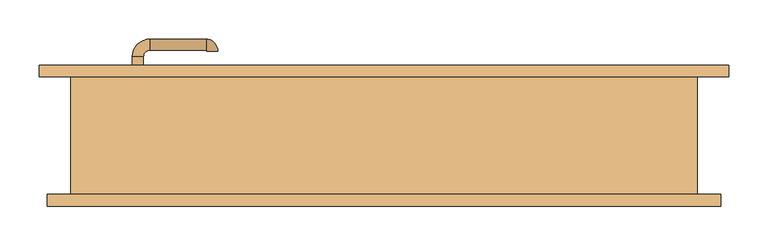
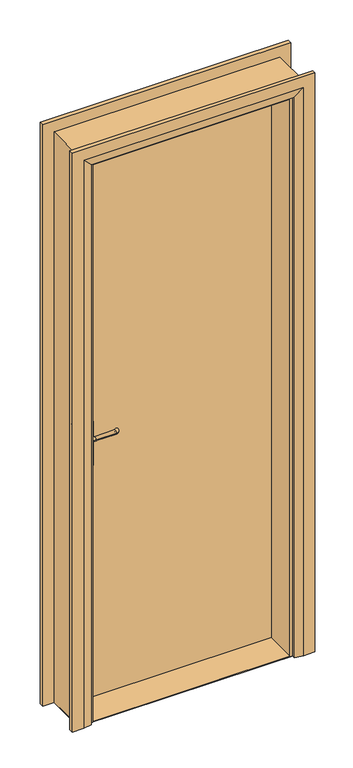
"""IFC4 building model written with IfcOpenShell, lengths in millimetres: door geometry, Porta Simples de Abrir : 70x210cm - Marco de Madeira."""

from ifc_helpers import new_model, si_unit, point, frame, frame_2d, origin, place, context, project, spatial, polyline, circle_curve, ellipse_curve, trimmed, segment, composite_curve, outline, extrude, faceted_brep, source, transform, mapped, element, save
from ifc_brep_helpers import plane_surface, cylinder_surface, revolved_surface, advanced_brep


def door_49983123(model_context):
    return source(origin(), model_context, "Body", "SolidModel", [
        extrude(outline(composite_curve([segment(trimmed(circle_curve(frame_2d((1050.0, -314.0)), 20.0), [point((1050.0, -334.0))], [point((1050.0, -294.0))], False, "CARTESIAN"), True, "CONTINUOUS"), segment(trimmed(circle_curve(frame_2d((1050.0, -314.0)), 20.0), [point((1050.0, -294.0))], [point((1050.0, -334.0))], False, "CARTESIAN"), True, "CONTINUOUS")], self_intersect=False)), frame((0.0, 29.4070105, 0.0), z_axis=(0.0, 1.0, 0.0), x_axis=(0.0, 0.0, 1.0)), (0.0, 0.0, 1.0), 4.5929895),
        advanced_brep(
        [(-307.0, 29.4070105, 1050.0), (-321.0, 29.4070105, 1050.0), (-321.0, 14.0, 1050.0), (-307.0, 14.0, 1050.0), (-299.0, -8.0, 1050.0), (-299.0, 6.0, 1050.0), (-227.0, -8.0, 1050.0), (-227.0, 6.0, 1050.0), (-226.0, 7.0, 1050.0), (-212.0, 7.0, 1050.0)],
        [
            (0, 1, circle_curve(frame((-314.0, 29.4070105, 1050.0), z_axis=(0.0, 1.0, 0.0), x_axis=(-1.0, 0.0, 0.0)), 7.0)),
            (1, 0, circle_curve(frame((-314.0, 29.4070105, 1050.0), z_axis=(0.0, 1.0, 0.0), x_axis=(-1.0, 0.0, 0.0)), 7.0)),
            (1, 2),
            (2, 3, circle_curve(frame((-314.0, 14.0, 1050.0), z_axis=(0.0, 1.0, 0.0), x_axis=(-1.0, 0.0, 0.0)), 7.0)),
            (3, 0),
            (3, 2, circle_curve(frame((-314.0, 14.0, 1050.0), z_axis=(0.0, 1.0, 0.0), x_axis=(-1.0, 0.0, 0.0)), 7.0)),
            (4, 5, circle_curve(frame((-299.0, -1.0, 1050.0), z_axis=(-1.0, 0.0, 0.0), x_axis=(0.0, -1.0, 0.0)), 7.0)),
            (5, 3, circle_curve(frame((-299.0, 14.0, 1050.0), z_axis=(0.0, 0.0, -1.0), x_axis=(-1.0, 0.0, 0.0)), 8.0)),
            (2, 4, circle_curve(frame((-299.0, 14.0, 1050.0), z_axis=(0.0, 0.0, 1.0), x_axis=(-1.0, 0.0, 0.0)), 22.0)),
            (5, 4, circle_curve(frame((-299.0, -1.0, 1050.0), z_axis=(-1.0, 0.0, 0.0), x_axis=(0.0, -1.0, 0.0)), 7.0)),
            (4, 6),
            (6, 7, circle_curve(frame((-227.0, -1.0, 1050.0), z_axis=(-1.0, 0.0, 0.0), x_axis=(0.0, -1.0, 0.0)), 7.0)),
            (7, 5),
            (7, 6, circle_curve(frame((-227.0, -1.0, 1050.0), z_axis=(-1.0, 0.0, 0.0), x_axis=(0.0, -1.0, 0.0)), 7.0)),
            (8, 9, circle_curve(frame((-219.0, 7.0, 1050.0), z_axis=(0.0, 1.0, 0.0), x_axis=(1.0, 0.0, 0.0)), 7.0)),
            (9, 8, circle_curve(frame((-219.0, 7.0, 1050.0), z_axis=(0.0, 1.0, 0.0), x_axis=(1.0, 0.0, 0.0)), 7.0)),
            (8, 7, circle_curve(frame((-227.0, 7.0, 1050.0), z_axis=(0.0, 0.0, -1.0), x_axis=(0.0, -1.0, 0.0)), 1.0)),
            (6, 9, circle_curve(frame((-227.0, 7.0, 1050.0), z_axis=(0.0, 0.0, 1.0), x_axis=(0.0, -1.0, 0.0)), 15.0)),
        ],
        [
            plane_surface(frame((-314.0, 29.4070105, 1050.0), z_axis=(0.0, 1.0, 0.0), x_axis=(0.0, 0.0, 1.0))),
            cylinder_surface(frame((-314.0, 29.4070105, 1050.0), z_axis=(0.0, 1.0, 0.0), x_axis=(-1.0, 0.0, 0.0)), 7.0),
            revolved_surface(trimmed(ellipse_curve(frame((-314.0, 14.0, 1050.0), z_axis=(0.0, -1.0, 0.0), x_axis=(-1.0, 0.0, 0.0)), 7.0, 7.0), [point((-307.0, 14.0, 1050.0))], [point((-321.0, 14.0, 1050.0))], True, "CARTESIAN"), (-299.0, 14.0, 1050.0), (0.0, 0.0, -1.0)),
            revolved_surface(trimmed(ellipse_curve(frame((-314.0, 14.0, 1050.0), z_axis=(0.0, -1.0, 0.0), x_axis=(-1.0, 0.0, 0.0)), 7.0, 7.0), [point((-321.0, 14.0, 1050.0))], [point((-307.0, 14.0, 1050.0))], True, "CARTESIAN"), (-299.0, 14.0, 1050.0), (0.0, 0.0, -1.0)),
            cylinder_surface(frame((-299.0, -1.0, 1050.0), z_axis=(-1.0, 0.0, 0.0), x_axis=(0.0, -1.0, 0.0)), 7.0),
            plane_surface(frame((-219.0, 7.0, 1050.0), z_axis=(0.0, 1.0, 0.0), x_axis=(0.0, 0.0, 1.0))),
            revolved_surface(trimmed(ellipse_curve(frame((-227.0, -1.0, 1050.0), z_axis=(1.0, 0.0, 0.0), x_axis=(0.0, -1.0, 0.0)), 7.0, 7.0), [point((-227.0, 6.0, 1050.0))], [point((-227.0, -8.0, 1050.0))], True, "CARTESIAN"), (-227.0, 7.0, 1050.0), (0.0, 0.0, -1.0)),
            revolved_surface(trimmed(ellipse_curve(frame((-227.0, -1.0, 1050.0), z_axis=(1.0, 0.0, 0.0), x_axis=(0.0, -1.0, 0.0)), 7.0, 7.0), [point((-227.0, -8.0, 1050.0))], [point((-227.0, 6.0, 1050.0))], True, "CARTESIAN"), (-227.0, 7.0, 1050.0), (0.0, 0.0, -1.0)),
        ],
        [
            (0, [[1, 2]]),
            (1, [[3, 4, 5, -2]]),
            (1, [[-5, 6, -3, -1]]),
            (2, [[7, 8, -4, 9]]),
            (3, [[10, -9, -6, -8]]),
            (4, [[11, 12, 13, -7]]),
            (4, [[-13, 14, -11, -10]]),
            (5, [[15, 16]]),
            (6, [[-15, 17, -12, 18]]),
            (7, [[-16, -18, -14, -17]]),
        ],
    ),
        extrude(outline(polyline([(-284.0, 40.0), (-284.0, 34.0), (-344.0, 34.0), (-344.0, 40.0), (-284.0, 40.0)])), frame((0.0, 0.0, 925.0), z_axis=(0.0, 0.0, 1.0), x_axis=(1.0, 0.0, 0.0)), (0.0, 0.0, 1.0), 165.0),
        extrude(outline(composite_curve([segment(trimmed(circle_curve(frame_2d((1050.0, -314.0)), 20.0), [point((1050.0, -334.0))], [point((1050.0, -294.0))], False, "CARTESIAN"), True, "CONTINUOUS"), segment(trimmed(circle_curve(frame_2d((1050.0, -314.0)), 20.0), [point((1050.0, -294.0))], [point((1050.0, -334.0))], False, "CARTESIAN"), True, "CONTINUOUS")], self_intersect=False)), frame((0.0, 81.0, 0.0), z_axis=(0.0, 1.0, 0.0), x_axis=(0.0, 0.0, 1.0)), (0.0, 0.0, 1.0), 4.5929895),
        advanced_brep(
        [(-307.0, 85.5929895, 1050.0), (-321.0, 85.5929895, 1050.0), (-307.0, 101.0, 1050.0), (-321.0, 101.0, 1050.0), (-299.0, 123.0, 1050.0), (-299.0, 109.0, 1050.0), (-227.0, 109.0, 1050.0), (-227.0, 123.0, 1050.0), (-226.0, 108.0, 1050.0), (-212.0, 108.0, 1050.0)],
        [
            (0, 1, circle_curve(frame((-314.0, 85.5929895, 1050.0), z_axis=(0.0, -1.0, 0.0), x_axis=(-1.0, 0.0, 0.0)), 7.0)),
            (1, 0, circle_curve(frame((-314.0, 85.5929895, 1050.0), z_axis=(0.0, -1.0, 0.0), x_axis=(-1.0, 0.0, 0.0)), 7.0)),
            (0, 2),
            (2, 3, circle_curve(frame((-314.0, 101.0, 1050.0), z_axis=(0.0, -1.0, 0.0), x_axis=(-1.0, 0.0, 0.0)), 7.0)),
            (3, 1),
            (3, 2, circle_curve(frame((-314.0, 101.0, 1050.0), z_axis=(0.0, -1.0, 0.0), x_axis=(-1.0, 0.0, 0.0)), 7.0)),
            (4, 3, circle_curve(frame((-299.0, 101.0, 1050.0), z_axis=(0.0, 0.0, 1.0), x_axis=(-1.0, 0.0, 0.0)), 22.0)),
            (2, 5, circle_curve(frame((-299.0, 101.0, 1050.0), z_axis=(0.0, 0.0, -1.0), x_axis=(-1.0, 0.0, 0.0)), 8.0)),
            (5, 4, circle_curve(frame((-299.0, 116.0, 1050.0), z_axis=(-1.0, 0.0, 0.0), x_axis=(0.0, 1.0, 0.0)), 7.0)),
            (4, 5, circle_curve(frame((-299.0, 116.0, 1050.0), z_axis=(-1.0, 0.0, 0.0), x_axis=(0.0, 1.0, 0.0)), 7.0)),
            (5, 6),
            (6, 7, circle_curve(frame((-227.0, 116.0, 1050.0), z_axis=(-1.0, 0.0, 0.0), x_axis=(0.0, 1.0, 0.0)), 7.0)),
            (7, 4),
            (7, 6, circle_curve(frame((-227.0, 116.0, 1050.0), z_axis=(-1.0, 0.0, 0.0), x_axis=(0.0, 1.0, 0.0)), 7.0)),
            (8, 9, circle_curve(frame((-219.0, 108.0, 1050.0), z_axis=(0.0, -1.0, 0.0), x_axis=(1.0, 0.0, 0.0)), 7.0)),
            (9, 8, circle_curve(frame((-219.0, 108.0, 1050.0), z_axis=(0.0, -1.0, 0.0), x_axis=(1.0, 0.0, 0.0)), 7.0)),
            (9, 7, circle_curve(frame((-227.0, 108.0, 1050.0), z_axis=(0.0, 0.0, 1.0), x_axis=(0.0, 1.0, 0.0)), 15.0)),
            (6, 8, circle_curve(frame((-227.0, 108.0, 1050.0), z_axis=(0.0, 0.0, -1.0), x_axis=(0.0, 1.0, 0.0)), 1.0)),
        ],
        [
            plane_surface(frame((-314.0, 85.5929895, 1050.0), z_axis=(0.0, -1.0, 0.0), x_axis=(0.0, 0.0, 1.0))),
            cylinder_surface(frame((-314.0, 85.5929895, 1050.0), z_axis=(0.0, -1.0, 0.0), x_axis=(-1.0, 0.0, 0.0)), 7.0),
            revolved_surface(trimmed(ellipse_curve(frame((-314.0, 101.0, 1050.0), z_axis=(0.0, -1.0, 0.0), x_axis=(-1.0, 0.0, 0.0)), 7.0, 7.0), [point((-307.0, 101.0, 1050.0))], [point((-321.0, 101.0, 1050.0))], True, "CARTESIAN"), (-299.0, 101.0, 1050.0), (0.0, 0.0, -1.0)),
            revolved_surface(trimmed(ellipse_curve(frame((-314.0, 101.0, 1050.0), z_axis=(0.0, -1.0, 0.0), x_axis=(-1.0, 0.0, 0.0)), 7.0, 7.0), [point((-321.0, 101.0, 1050.0))], [point((-307.0, 101.0, 1050.0))], True, "CARTESIAN"), (-299.0, 101.0, 1050.0), (0.0, 0.0, -1.0)),
            cylinder_surface(frame((-299.0, 116.0, 1050.0), z_axis=(-1.0, 0.0, 0.0), x_axis=(0.0, 1.0, 0.0)), 7.0),
            plane_surface(frame((-219.0, 108.0, 1050.0), z_axis=(0.0, -1.0, 0.0), x_axis=(0.0, 0.0, 1.0))),
            revolved_surface(trimmed(ellipse_curve(frame((-227.0, 116.0, 1050.0), z_axis=(-1.0, 0.0, 0.0), x_axis=(0.0, 1.0, 0.0)), 7.0, 7.0), [point((-227.0, 109.0, 1050.0))], [point((-227.0, 123.0, 1050.0))], True, "CARTESIAN"), (-227.0, 108.0, 1050.0), (0.0, 0.0, -1.0)),
            revolved_surface(trimmed(ellipse_curve(frame((-227.0, 116.0, 1050.0), z_axis=(-1.0, 0.0, 0.0), x_axis=(0.0, 1.0, 0.0)), 7.0, 7.0), [point((-227.0, 123.0, 1050.0))], [point((-227.0, 109.0, 1050.0))], True, "CARTESIAN"), (-227.0, 108.0, 1050.0), (0.0, 0.0, -1.0)),
        ],
        [
            (0, [[1, 2]]),
            (1, [[-1, 3, 4, 5]]),
            (1, [[-2, -5, 6, -3]]),
            (2, [[7, -4, 8, 9]]),
            (3, [[-8, -6, -7, 10]]),
            (4, [[-9, 11, 12, 13]]),
            (4, [[-10, -13, 14, -11]]),
            (5, [[15, 16]]),
            (6, [[17, -12, 18, -16]]),
            (7, [[-18, -14, -17, -15]]),
        ],
    ),
        extrude(outline(polyline([(-284.0, 75.0), (-344.0, 75.0), (-344.0, 81.0), (-284.0, 81.0), (-284.0, 75.0)])), frame((0.0, 0.0, 925.0), z_axis=(0.0, 0.0, 1.0), x_axis=(1.0, 0.0, 0.0)), (0.0, 0.0, 1.0), 165.0),
        extrude(outline(polyline([(358.0, 40.0), (-358.0, 40.0), (-358.0, 75.0), (358.0, 75.0), (358.0, 40.0)])), frame((0.0, 0.0, 53.0), z_axis=(0.0, 0.0, 1.0), x_axis=(1.0, 0.0, 0.0)), (0.0, 0.0, 1.0), 2094.0),
        faceted_brep([(430.0, -75.0, 50.0), (430.0, -90.0, 50.0), (390.0, -90.0, 50.0), (360.0, -85.0, 50.0), (360.0, -75.0, 50.0), (430.0, -75.0, 2220.0), (430.0, -90.0, 2220.0), (-430.0, -90.0, 2220.0), (-430.0, -90.0, 50.0), (-390.0, -90.0, 50.0), (-390.0, -90.0, 2180.0), (390.0, -90.0, 2180.0), (360.0, -85.0, 2150.0), (360.0, -75.0, 2150.0), (-360.0, -75.0, 2150.0), (-360.0, -75.0, 50.0), (-430.0, -75.0, 50.0), (-430.0, -75.0, 2220.0), (-360.0, -85.0, 2150.0), (-360.0, -85.0, 50.0)], [[[0, 1, 2, 3, 4]], [[1, 0, 5, 6]], [[2, 1, 6, 7, 8, 9, 10, 11]], [[3, 2, 11, 12]], [[4, 3, 12, 13]], [[0, 4, 13, 14, 15, 16, 17, 5]], [[14, 18, 19, 15]], [[16, 15, 19, 9, 8]], [[7, 17, 16, 8]], [[18, 10, 9, 19]], [[13, 12, 18, 14]], [[6, 5, 17, 7]], [[12, 11, 10, 18]]]),
        faceted_brep([(440.0, 75.0, 50.0), (370.0, 75.0, 50.0), (370.0, 85.0, 50.0), (400.0, 90.0, 50.0), (440.0, 90.0, 50.0), (440.0, 75.0, 2230.0), (-440.0, 75.0, 2230.0), (-440.0, 75.0, 50.0), (-370.0, 75.0, 50.0), (-370.0, 75.0, 2160.0), (370.0, 75.0, 2160.0), (370.0, 85.0, 2160.0), (400.0, 90.0, 2190.0), (-400.0, 90.0, 2190.0), (-400.0, 90.0, 50.0), (-440.0, 90.0, 50.0), (-440.0, 90.0, 2230.0), (440.0, 90.0, 2230.0), (-370.0, 85.0, 50.0), (-370.0, 85.0, 2160.0)], [[[0, 1, 2, 3, 4]], [[1, 0, 5, 6, 7, 8, 9, 10]], [[2, 1, 10, 11]], [[3, 2, 11, 12]], [[4, 3, 12, 13, 14, 15, 16, 17]], [[0, 4, 17, 5]], [[6, 16, 15, 7]], [[7, 15, 14, 18, 8]], [[19, 9, 8, 18]], [[13, 19, 18, 14]], [[11, 10, 9, 19]], [[5, 17, 16, 6]], [[12, 11, 19, 13]]]),
        faceted_brep([(-360.0, 75.0, 50.0), (-360.0, 38.0, 50.0), (-350.0, 38.0, 50.0), (-350.0, -75.0, 50.0), (-400.0, -75.0, 50.0), (-400.0, 75.0, 50.0), (-360.0, 75.0, 2150.0), (-360.0, 38.0, 2150.0), (-350.0, 38.0, 2140.0), (-350.0, -75.0, 2140.0), (-400.0, -75.0, 2190.0), (-400.0, 75.0, 2190.0), (360.0, 75.0, 50.0), (400.0, 75.0, 50.0), (400.0, -75.0, 50.0), (350.0, -75.0, 50.0), (350.0, 38.0, 50.0), (360.0, 38.0, 50.0), (360.0, 75.0, 2150.0), (400.0, 75.0, 2190.0), (400.0, -75.0, 2190.0), (350.0, -75.0, 2140.0), (350.0, 38.0, 2140.0), (360.0, 38.0, 2150.0)], [[[0, 1, 2, 3, 4, 5]], [[1, 0, 6, 7]], [[2, 1, 7, 8]], [[3, 2, 8, 9]], [[4, 3, 9, 10]], [[5, 4, 10, 11]], [[0, 5, 11, 6]], [[12, 13, 14, 15, 16, 17]], [[18, 19, 13, 12]], [[19, 20, 14, 13]], [[20, 21, 15, 14]], [[21, 22, 16, 15]], [[22, 23, 17, 16]], [[23, 18, 12, 17]], [[7, 6, 18, 23]], [[8, 7, 23, 22]], [[9, 8, 22, 21]], [[10, 9, 21, 20]], [[11, 10, 20, 19]], [[6, 11, 19, 18]]]),
        extrude(outline(polyline([(400.0, 40.0), (400.0, -75.0), (-400.0, -75.0), (-400.0, 40.0), (400.0, 40.0)])), frame((0.0, 0.0, 50.0), z_axis=(0.0, 0.0, 1.0), x_axis=(1.0, 0.0, 0.0)), (0.0, 0.0, 1.0), 3.0),
    ])


if __name__ == "__main__":
    model = new_model("IFC4")
    model_context = context("Model", 3, world=origin())
    ifc_project = project(units=[si_unit("LENGTHUNIT", "METRE", prefix="MILLI")], contexts=[model_context])
    site = spatial("IfcSite", under=ifc_project)
    building = spatial("IfcBuilding", under=site)
    placement = place(None, origin())
    door_shape = door_49983123(model_context)
    element("IfcDoor", 1, ObjectType="Porta Simples de Abrir : 70x210cm - Marco de Madeira", at=placement, inside=building, context=model_context, shape_type="MappedRepresentation", body=[
        mapped(door_shape, transform((0.0, 0.0, 0.0), x_axis=(1.0, 0.0, 0.0), y_axis=(0.0, 1.0, 0.0), z_axis=(0.0, 0.0, 1.0))),
    ])
    save(model, "model.ifc")

# Revit data of these elements
# Type "Porta Simples de Abrir : 70x210cm - Marco de Madeira"
#   Type Mark = "P58"
#   SINAPI = ""
#   Analytic Construction = "<Nenhum>"
#   Construction Type = "300"
#   Maçaneta [instance default] = ""
#   Fechadura [instance default] = ""
#   Vão Luz (somente para informação) = 0.680 m
#   Tolerância Folha Vertical = 0.003 m
#   Módulo Básico M = 0.100 m
#   Largura de Coordenação Modular Largura CM = 0.800 m
#   Rough Width = 0.800 m
#   Deslocamento da Horizontal da Folha = 0.000 m
#   Altura de Coordenação Modular Largura CM = 2.200 m
#   Rough Height = 2.200 m
#   Altura Nominal = 2.090 m
#   Ajuste de Coordenação Topo AC Topo = 0.010 m
#   Ajuste de Coordenação Base AC Base = 0.050 m
#   Ajuste de Coordenação AC = 0.010 m
#   Tolerância Folha Horizontal = 0.002 m
#   Largura Folha (somente para informação) = 0.696 m
#   Espessura Folha = 0.035 m
#   Maçaneta - Distância da Folha = 0.044 m
#   Maçaneta - Altura = 1.000 m
#   Largura Nominal (Largura Mn) = 0.720 m
#   Distância do Nível = 0.003 m
#   Aduela Interna Espessura = 0.040 m
#   Aduela Externa Espessura = 0.050 m
#   Altura Folha (somente para informação) = 2.075 m
#   Height = 2.140 m
#   Width = 0.780 m
#   Número de Módulos Básicos nM Largura = 8
#   Número de Módulos Básicos nM Altura = 22
#   Marco Metálico = no
#   Aduela de Madeira = no
#   Aduela Metálica de Canto = no
#   Guarnição Reta = no
#   Guarnição Chanfrada = yes
#   Batente - Material [instance default] = none
#   Painel - Material [instance default] = none
#   Model = ""
#   Function = (empty or 0)
#   Description = (empty or 0)
#   Wall Closure = (empty or 0)
#   Assembly Code = ""
# Element 1 (IfcDoor, "Porta Simples de Abrir : 70x210cm - Marco de Madeira")
#   Materials on its faces: "Porta - Maçaneta", "GRANITO"
# Materials
#   "Porta - Maçaneta": class "Diversos", colour RGB 0 0 0, transparency 0
#   "GRANITO": class "Genérico", colour RGB 120 120 120, transparency 0, Cost = 0
